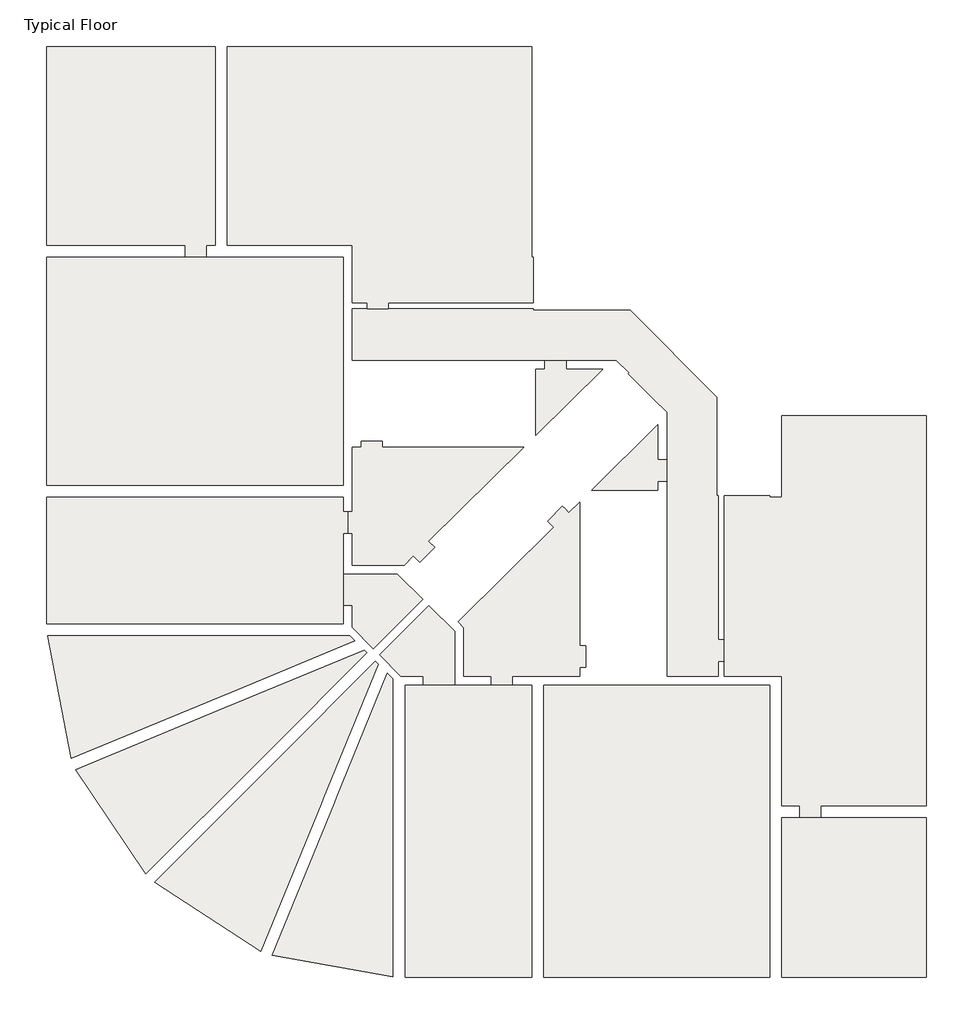
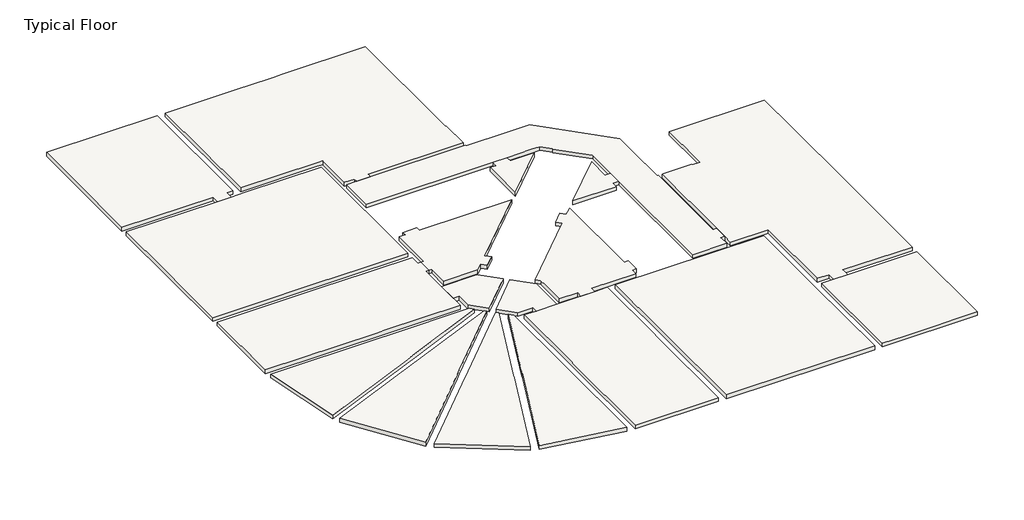
# One storey: 19 slabs.
"""IFC4 building model written with IfcOpenShell, lengths in millimetres."""

from ifc_helpers import new_model, si_unit, frame, origin, place, context, project, spatial, polyline, outline, extrude, faceted_brep, element, save

model = new_model("IFC4")

# Units and contexts
model_context = context("Model", 3, world=origin())
ifc_project = project(units=[si_unit("LENGTHUNIT", "METRE", prefix="MILLI")], contexts=[model_context])

# Site, building, storey
site = spatial("IfcSite", under=ifc_project)
building = spatial("IfcBuilding", under=site)
storey = spatial("IfcBuildingStorey", under=building, Name="Typical Floor", Elevation=3000.0)

# Slabs
placement = place(None, origin())
element("IfcSlab", 1, ObjectType="20", at=placement, inside=storey, context=model_context, shape_type="Brep", body=[
    faceted_brep([(-4461.7067397, 17456.8664083, 2800.0), (-4461.7067397, 9912.1590026, 2800.0), (-14296.6369988, 9912.1590026, 2800.0), (-14296.6369988, 17456.8664083, 2800.0), (-9693.3146493, 17456.8664083, 2800.0), (-9006.7279431, 17456.8664083, 2800.0), (-4461.7067397, 17456.8664083, 3000.0), (-8305.861308, 17456.8664083, 3000.0), (-9006.7279431, 17456.8664083, 3000.0), (-9693.3146493, 17456.8664083, 3000.0), (-14296.6369988, 17456.8664083, 3000.0), (-14296.6369988, 14107.3138675, 3000.0), (-14296.6369988, 13707.3138675, 3000.0), (-14296.6369988, 9912.1590026, 3000.0), (-8707.7294598, 9912.1590026, 3000.0), (-8307.7294598, 9912.1590026, 3000.0), (-4461.7067397, 9912.1590026, 3000.0)], [[[0, 1, 2, 3, 4, 5]], [[6, 7, 8, 9, 10, 11, 12, 13, 14, 15, 16]], [[1, 0, 6, 16]], [[2, 1, 16, 15, 14, 13]], [[3, 2, 13, 12, 11, 10]], [[0, 5, 4, 3, 10, 9, 8, 7, 6]]]),
])
element("IfcSlab", 2, ObjectType="20", at=placement, inside=storey, context=model_context, shape_type="SweptSolid", body=[
    extrude(outline(polyline([(-8705.861308, 24444.3058567), (-8705.861308, 17856.8664083), (-9006.7279431, 17856.8664083), (-9006.7279431, 17456.8664083), (-9693.3146493, 17456.8664083), (-9693.3146493, 17856.8664083), (-14296.6369988, 17856.8664083), (-14296.6369988, 24444.3058567), (-8705.861308, 24444.3058567)])), frame((0.0, 0.0, 2800.0), z_axis=(0.0, 0.0, 1.0), x_axis=(1.0, 0.0, 0.0)), (0.0, 0.0, 1.0), 200.0),
])
element("IfcSlab", 3, ObjectType="20", at=placement, inside=storey, context=model_context, shape_type="Brep", body=[
    faceted_brep([(1779.020722, 24445.393344, 2800.0), (1779.020722, 17856.8664083, 2800.0), (1779.020722, 17853.6134053, 2800.0), (1779.020722, 17453.6134053, 2800.0), (1829.020722, 17453.6134053, 2800.0), (1829.020722, 15961.3377606, 2800.0), (-2964.398431, 15961.3377606, 2800.0), (-2964.398431, 15761.3377606, 2800.0), (-3665.2660617, 15761.3377606, 2800.0), (-3665.2660617, 15961.3377606, 2800.0), (-4161.7067397, 15961.3377606, 2800.0), (-4161.7067397, 17856.8664083, 2800.0), (-4461.7067397, 17856.8664083, 2800.0), (-8305.861308, 17856.8664083, 2800.0), (-8305.861308, 24445.393344, 2800.0), (1779.020722, 17856.8664083, 3000.0), (1779.020722, 24445.393344, 3000.0), (-2413.8658054, 24445.393344, 3000.0), (-2813.8658054, 24445.393344, 3000.0), (-4118.3634455, 24445.393344, 3000.0), (-4518.3634455, 24445.393344, 3000.0), (-8305.861308, 24445.393344, 3000.0), (-8305.861308, 24444.3058567, 3000.0), (-8305.861308, 17856.8664083, 3000.0), (-4461.7067397, 17856.8664083, 3000.0), (-4161.7067397, 17856.8664083, 3000.0), (-4161.7067397, 15961.3377606, 3000.0), (-3665.2660617, 15961.3377606, 3000.0), (-3665.2660617, 15761.3377606, 3000.0), (-2964.398431, 15761.3377606, 3000.0), (-2964.398431, 15961.3377606, 3000.0), (1829.020722, 15961.3377606, 3000.0), (1829.020722, 16003.9996895, 3000.0), (1829.020722, 17453.6134053, 3000.0), (1779.020722, 17453.6134053, 3000.0), (1779.020722, 17853.6134053, 3000.0)], [[[0, 1, 2, 3, 4, 5, 6, 7, 8, 9, 10, 11, 12, 13, 14]], [[15, 16, 17, 18, 19, 20, 21, 22, 23, 24, 25, 26, 27, 28, 29, 30, 31, 32, 33, 34, 35]], [[1, 0, 16, 15]], [[1, 15, 35, 34, 3, 2]], [[4, 3, 34, 33]], [[5, 4, 33, 32, 31]], [[6, 5, 31, 30]], [[7, 6, 30, 29]], [[8, 7, 29, 28]], [[9, 8, 28, 27]], [[10, 9, 27, 26]], [[11, 10, 26, 25]], [[11, 25, 24, 23, 13, 12]], [[14, 13, 23, 22, 21]], [[0, 14, 21, 20, 19, 18, 17, 16]]]),
])
element("IfcSlab", 4, ObjectType="20", at=placement, inside=storey, context=model_context, shape_type="Brep", body=[
    faceted_brep([(-14296.6369988, 5319.511412, 2800.0), (-14296.6369988, 9512.1590026, 2800.0), (-4461.7067397, 9512.1590026, 2800.0), (-4461.7067397, 9032.3032318, 2800.0), (-4317.7621118, 9032.3032318, 2800.0), (-4317.7621118, 8319.3213117, 2800.0), (-4467.7621118, 8319.3213117, 2800.0), (-4467.7621118, 7259.3213117, 2800.0), (-4467.7621118, 6959.3213117, 2800.0), (-4467.7621118, 5921.5426188, 2800.0), (-4467.7621118, 5491.5426188, 2800.0), (-4467.7621118, 5319.511412, 2800.0), (-14296.6369988, 9512.1590026, 3000.0), (-14296.6369988, 5319.511412, 3000.0), (-8707.7294598, 5319.511412, 3000.0), (-8307.7294598, 5319.511412, 3000.0), (-4467.7621118, 5319.511412, 3000.0), (-4467.7621118, 5491.5426188, 3000.0), (-4467.7621118, 5921.5426188, 3000.0), (-4467.7621118, 6959.3213117, 3000.0), (-4467.7621118, 7259.3213117, 3000.0), (-4467.7621118, 8319.3213117, 3000.0), (-4317.7621118, 8319.3213117, 3000.0), (-4317.7621118, 9032.3032318, 3000.0), (-4461.7067397, 9032.3032318, 3000.0), (-4461.7067397, 9512.1590026, 3000.0), (-8307.7294598, 9512.1590026, 3000.0), (-8707.7294598, 9512.1590026, 3000.0)], [[[0, 1, 2, 3, 4, 5, 6, 7, 8, 9, 10, 11]], [[12, 13, 14, 15, 16, 17, 18, 19, 20, 21, 22, 23, 24, 25, 26, 27]], [[1, 0, 13, 12]], [[2, 1, 12, 27, 26, 25]], [[3, 2, 25, 24]], [[4, 3, 24, 23]], [[5, 4, 23, 22]], [[6, 5, 22, 21]], [[6, 21, 20, 19, 18, 9, 8, 7]], [[9, 18, 17, 16, 11, 10]], [[0, 11, 16, 15, 14, 13]]]),
])
element("IfcSlab", 5, ObjectType="20", at=placement, inside=storey, context=model_context, shape_type="Brep", body=[
    faceted_brep([(-4249.2842956, 4919.511412, 2800.0), (-4077.2097101, 4747.4368266, 2800.0), (-8177.5148344, 3048.7578016, 2800.0), (-8547.0578193, 2895.6631176, 2800.0), (-13484.0892311, 850.3441838, 2800.0), (-14261.3814687, 4919.511412, 2800.0), (-4077.2097101, 4747.4368266, 3000.0), (-4249.2842956, 4919.511412, 3000.0), (-8307.7294598, 4919.511412, 3000.0), (-8707.7294598, 4919.511412, 3000.0), (-14261.3814687, 4919.511412, 3000.0), (-13484.0892311, 850.3441838, 3000.0), (-8547.0578193, 2895.6631176, 3000.0), (-8177.5148344, 3048.7578016, 3000.0)], [[[0, 1, 2, 3, 4, 5]], [[6, 7, 8, 9, 10, 11, 12, 13]], [[1, 0, 7, 6]], [[1, 6, 13, 12, 11, 4, 3, 2]], [[5, 4, 11, 10]], [[0, 5, 10, 9, 8, 7]]]),
])
element("IfcSlab", 6, ObjectType="20", at=placement, inside=storey, context=model_context, shape_type="Brep", body=[
    faceted_brep([(-11001.7177394, -2970.8920309, 2800.0), (-13331.7826338, 480.4747094, 2800.0), (-8393.9631353, 2526.1201326, 2800.0), (-8024.4201504, 2679.2148167, 2800.0), (-3771.0702765, 4441.2973929, 2800.0), (-3680.299296, 4350.5264125, 2800.0), (-6954.3339133, 1076.4917952, 2800.0), (-7237.1766258, 793.6490827, 2800.0), (-13331.7826338, 480.4747094, 3000.0), (-11001.7177394, -2970.8920309, 3000.0), (-7237.1766258, 793.6490827, 3000.0), (-6954.3339133, 1076.4917952, 3000.0), (-3680.299296, 4350.5264125, 3000.0), (-3771.0702765, 4441.2973929, 3000.0), (-8024.4201504, 2679.2148167, 3000.0), (-8393.9631353, 2526.1201326, 3000.0)], [[[0, 1, 2, 3, 4, 5, 6, 7]], [[8, 9, 10, 11, 12, 13, 14, 15]], [[1, 0, 9, 8]], [[1, 8, 15, 14, 13, 4, 3, 2]], [[5, 4, 13, 12]], [[5, 12, 11, 10, 9, 0, 7, 6]]]),
])
element("IfcSlab", 7, ObjectType="20", at=placement, inside=storey, context=model_context, shape_type="Brep", body=[
    faceted_brep([(-3397.4447571, 4067.6718736, 2800.0), (-3302.3291451, 3972.5562616, 2800.0), (-5120.1129012, -471.1947368, 2800.0), (-5195.1092439, -649.6362255, 2800.0), (-5193.4008185, -650.3542517, 2800.0), (-7191.7801663, -5535.5889186, 2800.0), (-10715.1044827, -3249.987852, 2800.0), (-6954.3220945, 510.7945362, 2800.0), (-6671.4793821, 793.6372486, 2800.0), (-3302.3291451, 3972.5562616, 3000.0), (-3397.4447571, 4067.6718736, 3000.0), (-6671.4793821, 793.6372486, 3000.0), (-6954.3220945, 510.7945362, 3000.0), (-10715.1044827, -3249.987852, 3000.0), (-7191.7801663, -5535.5889186, 3000.0), (-5193.4008185, -650.3542517, 3000.0), (-5195.1092439, -649.6362255, 3000.0), (-5120.1129012, -471.1947368, 3000.0), (-5119.2358115, -469.0506048, 3000.0)], [[[0, 1, 2, 3, 4, 5, 6, 7, 8]], [[9, 10, 11, 12, 13, 14, 15, 16, 17, 18]], [[1, 0, 10, 9]], [[1, 9, 18, 17, 2]], [[14, 5, 4, 15]], [[6, 5, 14, 13]], [[6, 13, 12, 11, 10, 0, 8, 7]], [[3, 16, 15, 4]], [[16, 3, 2, 17]]]),
])
element("IfcSlab", 8, ObjectType="20", at=placement, inside=storey, context=model_context, shape_type="Brep", body=[
    faceted_brep([(-2813.8658054, 3484.0929218, 2800.0), (-2813.8658054, -6379.2217224, 2800.0), (-6818.4727302, -5679.49154, 2800.0), (-4750.6157411, -624.4119522, 2800.0), (-4671.3715454, -435.8633948, 2800.0), (-4673.1767374, -435.1046991, 2800.0), (-2995.6201329, 3665.8472494, 2800.0), (-2909.1120413, 3579.3391577, 2800.0), (-2813.8658054, -6379.2217224, 3000.0), (-2813.8658054, -1123.2844162, 3000.0), (-2813.8658054, -723.2844162, 3000.0), (-2813.8658054, 3484.0929218, 3000.0), (-2909.1120413, 3579.3391577, 3000.0), (-2995.6201329, 3665.8472494, 3000.0), (-4673.1767374, -435.1046991, 3000.0), (-4671.3715454, -435.8633948, 3000.0), (-4750.6157411, -624.4119522, 3000.0), (-6818.4727302, -5679.49154, 3000.0)], [[[0, 1, 2, 3, 4, 5, 6, 7]], [[8, 9, 10, 11, 12, 13, 14, 15, 16, 17]], [[1, 0, 11, 10, 9, 8]], [[2, 1, 8, 17]], [[13, 6, 5, 14]], [[2, 17, 16, 3]], [[6, 13, 12, 11, 0, 7]], [[4, 15, 14, 5]], [[15, 4, 3, 16]]]),
])
element("IfcSlab", 9, ObjectType="20", at=placement, inside=storey, context=model_context, shape_type="Brep", body=[
    faceted_brep([(1779.020722, 3279.3391577, 2800.0), (1779.020722, -6410.076772, 2800.0), (-2413.8658054, -6410.076772, 2800.0), (-2413.8658054, 3279.3391577, 2800.0), (-1817.5239543, 3279.3391577, 2800.0), (-769.9852407, 3279.3391577, 2800.0), (450.0147593, 3279.3391577, 2800.0), (1134.6168888, 3279.3391577, 2800.0), (1779.020722, 3279.3391577, 3000.0), (1134.6168888, 3279.3391577, 3000.0), (450.0147593, 3279.3391577, 3000.0), (-469.9852407, 3279.3391577, 3000.0), (-769.9852407, 3279.3391577, 3000.0), (-1817.5239543, 3279.3391577, 3000.0), (-2413.8658054, 3279.3391577, 3000.0), (-2413.8658054, -723.2844162, 3000.0), (-2413.8658054, -1123.2844162, 3000.0), (-2413.8658054, -6410.076772, 3000.0), (1779.020722, -6410.076772, 3000.0), (1779.020722, -1123.2844162, 3000.0), (1779.020722, -723.2844162, 3000.0)], [[[0, 1, 2, 3, 4, 5, 6, 7]], [[8, 9, 10, 11, 12, 13, 14, 15, 16, 17, 18, 19, 20]], [[1, 0, 8, 20, 19, 18]], [[2, 1, 18, 17]], [[3, 2, 17, 16, 15, 14]], [[0, 7, 6, 5, 4, 3, 14, 13, 12, 11, 10, 9, 8]]]),
])
element("IfcSlab", 10, ObjectType="20", at=placement, inside=storey, context=model_context, shape_type="Brep", body=[
    faceted_brep([(9669.6339123, 3279.3391577, 2800.0), (9669.6339123, -6410.076772, 2800.0), (2179.020722, -6410.076772, 2800.0), (2179.020722, 3279.3391577, 2800.0), (9669.6339123, 3279.3391577, 3000.0), (2179.020722, 3279.3391577, 3000.0), (2179.020722, -723.2844162, 3000.0), (2179.020722, -1123.2844162, 3000.0), (2179.020722, -6410.076772, 3000.0), (5922.4147884, -6410.076772, 3000.0), (6322.4147884, -6410.076772, 3000.0), (9669.6339123, -6410.076772, 3000.0), (9669.6339123, -1116.1309652, 3000.0), (9669.6339123, -716.1309652, 3000.0)], [[[0, 1, 2, 3]], [[4, 5, 6, 7, 8, 9, 10, 11, 12, 13]], [[1, 0, 4, 13, 12, 11]], [[2, 1, 11, 10, 9, 8]], [[3, 2, 8, 7, 6, 5]], [[0, 3, 5, 4]]]),
])
element("IfcSlab", 11, ObjectType="20", at=placement, inside=storey, context=model_context, shape_type="Brep", body=[
    faceted_brep([(14862.6652109, -1116.1309652, 2800.0), (14862.6652109, -6410.076772, 2800.0), (10069.6339123, -6410.076772, 2800.0), (10069.6339123, -1116.1309652, 2800.0), (10670.3228524, -1116.1309652, 2800.0), (11362.6652109, -1116.1309652, 2800.0), (14862.6652109, -1116.1309652, 3000.0), (11362.6652109, -1116.1309652, 3000.0), (10670.3228524, -1116.1309652, 3000.0), (10069.6339123, -1116.1309652, 3000.0), (10069.6339123, -6410.076772, 3000.0), (11162.4147884, -6410.076772, 3000.0), (14862.6652109, -6410.076772, 3000.0)], [[[0, 1, 2, 3, 4, 5]], [[6, 7, 8, 9, 10, 11, 12]], [[1, 0, 6, 12]], [[2, 1, 12, 11, 10]], [[3, 2, 10, 9]], [[0, 5, 4, 3, 9, 8, 7, 6]]]),
])
element("IfcSlab", 12, ObjectType="20", at=placement, inside=storey, context=model_context, shape_type="Brep", body=[
    faceted_brep([(10670.3228524, -716.1309652, 2800.0), (10069.6339123, -716.1309652, 2800.0), (10069.6339123, 3279.3391577, 2800.0), (10069.6339123, 3579.3391577, 2800.0), (8168.0773416, 3579.3391577, 2800.0), (8168.0773416, 4078.4432768, 2800.0), (8168.0773416, 4779.3109075, 2800.0), (8168.0773416, 9562.1590026, 2800.0), (8219.6339123, 9562.1590026, 2800.0), (9669.6339123, 9562.1590026, 2800.0), (9669.6339123, 9512.1590026, 2800.0), (10069.6339123, 9512.1590026, 2800.0), (10069.6339123, 9912.1590026, 2800.0), (10069.6339123, 12213.3492909, 2800.0), (14862.3806142, 12213.3492909, 2800.0), (14862.3806142, -716.1309652, 2800.0), (11362.6652109, -716.1309652, 2800.0), (11362.6652109, -1116.1309652, 2800.0), (10670.3228524, -1116.1309652, 2800.0), (10069.6339123, -716.1309652, 3000.0), (10670.3228524, -716.1309652, 3000.0), (10670.3228524, -1116.1309652, 3000.0), (11362.6652109, -1116.1309652, 3000.0), (11362.6652109, -716.1309652, 3000.0), (14862.3806142, -716.1309652, 3000.0), (14862.3806142, 3228.4489922, 3000.0), (14862.3806142, 3628.4489922, 3000.0), (14862.3806142, 4919.511412, 3000.0), (14862.3806142, 5319.511412, 3000.0), (14862.3806142, 9512.1590026, 3000.0), (14862.3806142, 9912.1590026, 3000.0), (14862.3806142, 12213.3492909, 3000.0), (10069.6339123, 12213.3492909, 3000.0), (10069.6339123, 9912.1590026, 3000.0), (10069.6339123, 9512.1590026, 3000.0), (9669.6339123, 9512.1590026, 3000.0), (9669.6339123, 9562.1590026, 3000.0), (8219.6339123, 9562.1590026, 3000.0), (8168.0773416, 9562.1590026, 3000.0), (8168.0773416, 4779.3109075, 3000.0), (8168.0773416, 4078.4432768, 3000.0), (8168.0773416, 3579.3391577, 3000.0), (10069.6339123, 3579.3391577, 3000.0), (10069.6339123, 3279.3391577, 3000.0)], [[[0, 1, 2, 3, 4, 5, 6, 7, 8, 9, 10, 11, 12, 13, 14, 15, 16, 17, 18]], [[19, 20, 21, 22, 23, 24, 25, 26, 27, 28, 29, 30, 31, 32, 33, 34, 35, 36, 37, 38, 39, 40, 41, 42, 43]], [[1, 0, 20, 19]], [[1, 19, 43, 42, 3, 2]], [[4, 3, 42, 41]], [[6, 5, 4, 41, 40, 39]], [[7, 6, 39, 38]], [[7, 38, 37, 36, 9, 8]], [[10, 9, 36, 35]], [[11, 10, 35, 34]], [[11, 34, 33, 32, 13, 12]], [[14, 13, 32, 31]], [[15, 14, 31, 30, 29, 28, 27, 26, 25, 24]], [[16, 15, 24, 23]], [[17, 16, 23, 22]], [[18, 17, 22, 21]], [[0, 18, 21, 20]]]),
])
element("IfcSlab", 13, ObjectType="20", at=placement, inside=storey, context=model_context, shape_type="SweptSolid", body=[
    extrude(outline(polyline([(-769.9852407, 5064.4841024), (-769.9852407, 3279.3391577), (-1817.5239543, 3279.3391577), (-1817.5239543, 3579.3391577), (-2555.5586507, 3579.3391577), (-3256.6787431, 4280.4592501), (-1621.3195657, 5915.8184274), (-769.9852407, 5064.4841024)])), frame((0.0, 0.0, 2800.0), z_axis=(0.0, 0.0, 1.0), x_axis=(1.0, 0.0, 0.0)), (0.0, 0.0, 1.0), 200.0),
])
element("IfcSlab", 14, ObjectType="20", at=placement, inside=storey, context=model_context, shape_type="Brep", body=[
    faceted_brep([(-2664.82245, 6959.3213117, 2800.0), (-1833.4516001, 6127.9504618, 2800.0), (-3468.8107774, 4492.5912844, 2800.0), (-4167.7621118, 5191.5426188, 2800.0), (-4167.7621118, 5921.5426188, 2800.0), (-4467.7621118, 5921.5426188, 2800.0), (-4467.7621118, 6959.3213117, 2800.0), (-1833.4516001, 6127.9504618, 3000.0), (-2664.82245, 6959.3213117, 3000.0), (-2752.523137, 6959.3213117, 3000.0), (-4467.7621118, 6959.3213117, 3000.0), (-4467.7621118, 5921.5426188, 3000.0), (-4167.7621118, 5921.5426188, 3000.0), (-4167.7621118, 5191.5426188, 3000.0), (-3468.8107774, 4492.5912844, 3000.0)], [[[0, 1, 2, 3, 4, 5, 6]], [[7, 8, 9, 10, 11, 12, 13, 14]], [[1, 0, 8, 7]], [[2, 1, 7, 14]], [[3, 2, 14, 13]], [[4, 3, 13, 12]], [[5, 4, 12, 11]], [[6, 5, 11, 10]], [[0, 6, 10, 9, 8]]]),
])
element("IfcSlab", 15, ObjectType="20", at=placement, inside=storey, context=model_context, shape_type="SweptSolid", body=[
    extrude(outline(polyline([(-4317.7621118, 9032.3032318), (-4161.7067397, 9032.3032318), (-4161.7067397, 11166.7645142), (-3861.7208648, 11166.7645142), (-3861.7208648, 11366.7645142), (-3166.1629714, 11366.7645142), (-3166.1629714, 11166.7645142), (1521.6521635, 11166.7645142), (-1638.9943721, 8055.4647086), (-1428.5378745, 7841.6702684), (-1923.597057, 7354.3403753), (-2134.0535546, 7568.1348155), (-2447.7649909, 7259.3213117), (-4167.7621118, 7259.3213117), (-4167.7621118, 8319.3213117), (-4317.7621118, 8319.3213117), (-4317.7621118, 9032.3032318)])), frame((0.0, 0.0, 2800.0), z_axis=(0.0, 0.0, 1.0), x_axis=(1.0, 0.0, 0.0)), (0.0, 0.0, 1.0), 200.0),
])
element("IfcSlab", 16, ObjectType="20", at=placement, inside=storey, context=model_context, shape_type="Brep", body=[
    faceted_brep([(450.0147593, 3579.3391577, 2800.0), (-469.9852407, 3579.3391577, 2800.0), (-469.9852407, 4764.4841024, 2800.0), (-469.9852407, 5188.7481711, 2800.0), (-654.972774, 5373.7357044, 2800.0), (2521.8013373, 8504.6910362, 2800.0), (2309.6637065, 8716.8286669, 2800.0), (2804.6384533, 9211.8034138, 2800.0), (2897.8940684, 9118.5477987, 2800.0), (3019.4754557, 8995.1871747, 2800.0), (3020.3715361, 8996.0703309, 2800.0), (3375.2686355, 9345.8487309, 2800.0), (3375.2686355, 4577.5453716, 2800.0), (3575.2686355, 4577.5453716, 2800.0), (3575.2686355, 3876.6777409, 2800.0), (3375.2686355, 3876.6777409, 2800.0), (3375.2686355, 3579.3391577, 2800.0), (1134.6168888, 3579.3391577, 2800.0), (1134.6168888, 3279.3391577, 2800.0), (450.0147593, 3279.3391577, 2800.0), (-469.9852407, 3579.3391577, 3000.0), (450.0147593, 3579.3391577, 3000.0), (450.0147593, 3279.3391577, 3000.0), (1134.6168888, 3279.3391577, 3000.0), (1134.6168888, 3579.3391577, 3000.0), (3375.2686355, 3579.3391577, 3000.0), (3375.2686355, 3876.6777409, 3000.0), (3575.2686355, 3876.6777409, 3000.0), (3575.2686355, 4577.5453716, 3000.0), (3375.2686355, 4577.5453716, 3000.0), (3375.2686355, 9345.8487309, 3000.0), (3020.3715361, 8996.0703309, 3000.0), (3019.4754557, 8995.1871747, 3000.0), (2897.8940684, 9118.5477987, 3000.0), (2804.6384533, 9211.8034138, 3000.0), (2309.6637065, 8716.8286669, 3000.0), (2521.8013373, 8504.6910362, 3000.0), (-654.972774, 5373.7357044, 3000.0), (-469.9852407, 5188.7481711, 3000.0), (-469.9852407, 4764.4841024, 3000.0)], [[[0, 1, 2, 3, 4, 5, 6, 7, 8, 9, 10, 11, 12, 13, 14, 15, 16, 17, 18, 19]], [[20, 21, 22, 23, 24, 25, 26, 27, 28, 29, 30, 31, 32, 33, 34, 35, 36, 37, 38, 39]], [[1, 0, 21, 20]], [[1, 20, 39, 38, 3, 2]], [[4, 3, 38, 37]], [[5, 4, 37, 36]], [[6, 5, 36, 35]], [[7, 6, 35, 34]], [[7, 34, 33, 8]], [[29, 12, 11, 30]], [[13, 12, 29, 28]], [[14, 13, 28, 27]], [[15, 14, 27, 26]], [[16, 15, 26, 25]], [[17, 16, 25, 24]], [[18, 17, 24, 23]], [[19, 18, 23, 22]], [[0, 19, 22, 21]], [[9, 32, 31, 30, 11, 10]], [[32, 9, 8, 33]]]),
])
element("IfcSlab", 17, ObjectType="20", at=placement, inside=storey, context=model_context, shape_type="SweptSolid", body=[
    extrude(outline(polyline([(1924.8242608, 13749.3760398), (2223.0854171, 13749.3760398), (2223.0854171, 14049.3760398), (2926.3637213, 14049.3760398), (2926.3637213, 13749.3760398), (4145.2251653, 13749.3760398), (1924.8242608, 11563.6419424), (1924.8242608, 13749.3760398)])), frame((0.0, 0.0, 2800.0), z_axis=(0.0, 0.0, 1.0), x_axis=(1.0, 0.0, 0.0)), (0.0, 0.0, 1.0), 200.0),
])
element("IfcSlab", 18, ObjectType="20", at=placement, inside=storey, context=model_context, shape_type="SweptSolid", body=[
    extrude(outline(polyline([(5969.003497, 11902.1740186), (5969.003497, 10741.9965509), (6269.003497, 10741.9965509), (6269.003497, 10041.1289202), (5969.003497, 10041.1289202), (5969.003497, 9742.8632028), (3778.0930653, 9742.8632028), (5969.003497, 11902.1740186)])), frame((0.0, 0.0, 2800.0), z_axis=(0.0, 0.0, 1.0), x_axis=(1.0, 0.0, 0.0)), (0.0, 0.0, 1.0), 200.0),
])
element("IfcSlab", 19, ObjectType="20", at=placement, inside=storey, context=model_context, shape_type="Brep", body=[
    faceted_brep([(7968.0773416, 3579.3391577, 2800.0), (6269.003497, 3579.3391577, 2800.0), (6269.003497, 10041.1289202, 2800.0), (6269.003497, 10741.9965509, 2800.0), (6269.003497, 11899.9963547, 2800.0), (6269.003497, 12324.2604234, 2800.0), (5836.2714262, 12756.9924943, 2800.0), (4989.3898697, 13603.8740507, 2800.0), (5010.62779, 13625.111971, 2800.0), (4586.3637213, 14049.3760398, 2800.0), (4162.0996526, 14049.3760398, 2800.0), (2926.3637213, 14049.3760398, 2800.0), (2223.0854171, 14049.3760398, 2800.0), (-4161.7067397, 14049.3760398, 2800.0), (-4161.7067397, 15761.3377606, 2800.0), (-3665.2660617, 15761.3377606, 2800.0), (-2964.398431, 15761.3377606, 2800.0), (1829.020722, 15761.3377606, 2800.0), (1829.020722, 15703.9996895, 2800.0), (2129.020722, 15703.9996895, 2800.0), (3673.883474, 15703.9996895, 2800.0), (3973.883474, 15703.9996895, 2800.0), (5042.5813574, 15703.9996895, 2800.0), (7919.6339123, 12826.9471346, 2800.0), (7919.6339123, 11715.5910733, 2800.0), (7919.6339123, 11415.5910733, 2800.0), (7919.6339123, 9862.1590026, 2800.0), (7919.6339123, 9562.1590026, 2800.0), (7968.0773416, 9562.1590026, 2800.0), (7968.0773416, 4779.3109075, 2800.0), (8168.0773416, 4779.3109075, 2800.0), (8168.0773416, 4078.4432768, 2800.0), (7968.0773416, 4078.4432768, 2800.0), (6269.003497, 3579.3391577, 3000.0), (7968.0773416, 3579.3391577, 3000.0), (7968.0773416, 4078.4432768, 3000.0), (8168.0773416, 4078.4432768, 3000.0), (8168.0773416, 4779.3109075, 3000.0), (7968.0773416, 4779.3109075, 3000.0), (7968.0773416, 9562.1590026, 3000.0), (7919.6339123, 9562.1590026, 3000.0), (7919.6339123, 9862.1590026, 3000.0), (7919.6339123, 11415.5910733, 3000.0), (7919.6339123, 11715.5910733, 3000.0), (7919.6339123, 12826.9471346, 3000.0), (5042.5813574, 15703.9996895, 3000.0), (3973.883474, 15703.9996895, 3000.0), (3673.883474, 15703.9996895, 3000.0), (2129.020722, 15703.9996895, 3000.0), (1829.020722, 15703.9996895, 3000.0), (1829.020722, 15761.3377606, 3000.0), (-2964.398431, 15761.3377606, 3000.0), (-3665.2660617, 15761.3377606, 3000.0), (-4161.7067397, 15761.3377606, 3000.0), (-4161.7067397, 14049.3760398, 3000.0), (2223.0854171, 14049.3760398, 3000.0), (2926.3637213, 14049.3760398, 3000.0), (4162.0996526, 14049.3760398, 3000.0), (4586.3637213, 14049.3760398, 3000.0), (5010.62779, 13625.111971, 3000.0), (4989.3898697, 13603.8740507, 3000.0), (5836.2714262, 12756.9924943, 3000.0), (6269.003497, 12324.2604234, 3000.0), (6269.003497, 11899.9963547, 3000.0), (6269.003497, 10741.9965509, 3000.0), (6269.003497, 10041.1289202, 3000.0)], [[[0, 1, 2, 3, 4, 5, 6, 7, 8, 9, 10, 11, 12, 13, 14, 15, 16, 17, 18, 19, 20, 21, 22, 23, 24, 25, 26, 27, 28, 29, 30, 31, 32]], [[33, 34, 35, 36, 37, 38, 39, 40, 41, 42, 43, 44, 45, 46, 47, 48, 49, 50, 51, 52, 53, 54, 55, 56, 57, 58, 59, 60, 61, 62, 63, 64, 65]], [[1, 0, 34, 33]], [[1, 33, 65, 64, 63, 62, 5, 4, 3, 2]], [[5, 62, 61, 60, 7, 6]], [[8, 7, 60, 59]], [[9, 8, 59, 58]], [[9, 58, 57, 56, 55, 54, 13, 12, 11, 10]], [[14, 13, 54, 53]], [[17, 16, 15, 14, 53, 52, 51, 50]], [[18, 17, 50, 49]], [[18, 49, 48, 47, 46, 45, 22, 21, 20, 19]], [[40, 27, 26, 25, 24, 23, 44, 43, 42, 41]], [[28, 27, 40, 39]], [[29, 28, 39, 38]], [[23, 22, 45, 44]], [[30, 29, 38, 37]], [[31, 30, 37, 36]], [[32, 31, 36, 35]], [[0, 32, 35, 34]]]),
])

save(model, "model.ifc")

# Revit data of these elements
# Type "20"
#   Function = 0
#   Layers, outside or top first: 20 cm "Concrete" (function 1)
# Element 1 (IfcSlab, "20")
#   Mark = "S1"
#   SOFiSTiK_AMG_Comments = ""
#   Height Offset From Level = 0 cm
#   built-in parameter 1001954 = 1
#   SOFiSTiK_AMG_Scheduled = yes
#   SOFiSTiK_AMG_Adjusted = yes
#   Phase Created = New Construction
#   Materials on its faces: "Concrete"
# Element 2 (IfcSlab, "20")
#   Mark = "S2"
#   SOFiSTiK_AMG_Comments = ""
#   Height Offset From Level = 0 cm
#   built-in parameter 1001954 = 1
#   SOFiSTiK_AMG_Scheduled = yes
#   SOFiSTiK_AMG_Adjusted = yes
#   Phase Created = New Construction
#   Materials on its faces: "Concrete"
# Element 3 (IfcSlab, "20")
#   Mark = "S3"
#   SOFiSTiK_AMG_Comments = ""
#   Height Offset From Level = 0 cm
#   built-in parameter 1001954 = 1
#   SOFiSTiK_AMG_Scheduled = yes
#   SOFiSTiK_AMG_Adjusted = yes
#   Phase Created = New Construction
#   Materials on its faces: "Concrete"
# Element 4 (IfcSlab, "20")
#   Mark = "S4"
#   SOFiSTiK_AMG_Comments = ""
#   built-in parameter 1001955 = -1.5708 (stored number, unit not read)
#   Height Offset From Level = 0 cm
#   built-in parameter 1001954 = 1
#   SOFiSTiK_AMG_Scheduled = yes
#   SOFiSTiK_AMG_Adjusted = yes
#   Phase Created = New Construction
#   Materials on its faces: "Concrete"
# Element 5 (IfcSlab, "20")
#   Mark = "S5"
#   SOFiSTiK_AMG_Comments = ""
#   Height Offset From Level = 0 cm
#   built-in parameter 1001954 = 1
#   SOFiSTiK_AMG_Scheduled = yes
#   SOFiSTiK_AMG_Adjusted = yes
#   Phase Created = New Construction
#   Materials on its faces: "Concrete"
# Element 6 (IfcSlab, "20")
#   Mark = "S6"
#   SOFiSTiK_AMG_Comments = ""
#   built-in parameter 1001955 = -0.976969 (stored number, unit not read)
#   Height Offset From Level = 0 cm
#   built-in parameter 1001954 = 1
#   SOFiSTiK_AMG_Scheduled = yes
#   SOFiSTiK_AMG_Adjusted = yes
#   Phase Created = New Construction
#   Materials on its faces: "Concrete"
# Element 7 (IfcSlab, "20")
#   Mark = "S7"
#   SOFiSTiK_AMG_Comments = ""
#   built-in parameter 1001955 = 2.35619 (stored number, unit not read)
#   Height Offset From Level = 0 cm
#   built-in parameter 1001954 = 1
#   SOFiSTiK_AMG_Scheduled = yes
#   SOFiSTiK_AMG_Adjusted = yes
#   Phase Created = New Construction
#   Materials on its faces: "Concrete"
# Element 8 (IfcSlab, "20")
#   Mark = "S8"
#   SOFiSTiK_AMG_Comments = ""
#   built-in parameter 1001955 = -0.785398 (stored number, unit not read)
#   Height Offset From Level = 0 cm
#   built-in parameter 1001954 = 1
#   SOFiSTiK_AMG_Scheduled = yes
#   SOFiSTiK_AMG_Adjusted = yes
#   Phase Created = New Construction
#   Materials on its faces: "Concrete"
# Element 9 (IfcSlab, "20")
#   Mark = "S9"
#   SOFiSTiK_AMG_Comments = ""
#   Height Offset From Level = 0 cm
#   built-in parameter 1001954 = 1
#   SOFiSTiK_AMG_Scheduled = yes
#   SOFiSTiK_AMG_Adjusted = yes
#   Phase Created = New Construction
#   Materials on its faces: "Concrete"
# Element 10 (IfcSlab, "20")
#   Mark = "S10"
#   SOFiSTiK_AMG_Comments = ""
#   Height Offset From Level = 0 cm
#   built-in parameter 1001954 = 1
#   SOFiSTiK_AMG_Scheduled = yes
#   SOFiSTiK_AMG_Adjusted = yes
#   Phase Created = New Construction
#   Materials on its faces: "Concrete"
# Element 11 (IfcSlab, "20")
#   Mark = "S11"
#   SOFiSTiK_AMG_Comments = ""
#   Height Offset From Level = 0 cm
#   built-in parameter 1001954 = 1
#   SOFiSTiK_AMG_Scheduled = yes
#   SOFiSTiK_AMG_Adjusted = yes
#   Phase Created = New Construction
#   Materials on its faces: "Concrete"
# Element 12 (IfcSlab, "20")
#   Mark = "S12"
#   SOFiSTiK_AMG_Comments = ""
#   built-in parameter 1001955 = 1.5708 (stored number, unit not read)
#   Height Offset From Level = 0 cm
#   built-in parameter 1001954 = 1
#   SOFiSTiK_AMG_Scheduled = yes
#   SOFiSTiK_AMG_Adjusted = no
#   Phase Created = New Construction
#   Materials on its faces: "Concrete"
# Element 13 (IfcSlab, "20")
#   Mark = "S13"
#   SOFiSTiK_AMG_Comments = ""
#   built-in parameter 1001955 = 1.5708 (stored number, unit not read)
#   Height Offset From Level = 0 cm
#   built-in parameter 1001954 = 1
#   SOFiSTiK_AMG_Scheduled = yes
#   SOFiSTiK_AMG_Adjusted = yes
#   Phase Created = New Construction
#   Materials on its faces: "Concrete"
# Element 14 (IfcSlab, "20")
#   Mark = "S14"
#   SOFiSTiK_AMG_Comments = ""
#   Height Offset From Level = 0 cm
#   built-in parameter 1001954 = 1
#   SOFiSTiK_AMG_Scheduled = yes
#   SOFiSTiK_AMG_Adjusted = yes
#   Phase Created = New Construction
#   Materials on its faces: "Concrete"
# Element 15 (IfcSlab, "20")
#   Mark = "S15"
#   SOFiSTiK_AMG_Comments = ""
#   built-in parameter 1001955 = 1.5708 (stored number, unit not read)
#   Height Offset From Level = 0 cm
#   built-in parameter 1001954 = 1
#   SOFiSTiK_AMG_Scheduled = yes
#   SOFiSTiK_AMG_Adjusted = yes
#   Phase Created = New Construction
#   Materials on its faces: "Concrete"
# Element 16 (IfcSlab, "20")
#   Mark = "S16"
#   SOFiSTiK_AMG_Comments = ""
#   built-in parameter 1001955 = 1.5708 (stored number, unit not read)
#   Height Offset From Level = 0 cm
#   built-in parameter 1001954 = 1
#   SOFiSTiK_AMG_Scheduled = yes
#   SOFiSTiK_AMG_Adjusted = yes
#   Phase Created = New Construction
#   Materials on its faces: "Concrete"
# Element 17 (IfcSlab, "20")
#   Mark = "S17"
#   SOFiSTiK_AMG_Comments = ""
#   built-in parameter 1001955 = 0.77753 (stored number, unit not read)
#   Height Offset From Level = 0 cm
#   built-in parameter 1001954 = 1
#   SOFiSTiK_AMG_Scheduled = yes
#   SOFiSTiK_AMG_Adjusted = yes
#   Phase Created = New Construction
#   Materials on its faces: "Concrete"
# Element 18 (IfcSlab, "20")
#   Mark = "S18"
#   SOFiSTiK_AMG_Comments = ""
#   built-in parameter 1001955 = 0.778134 (stored number, unit not read)
#   Height Offset From Level = 0 cm
#   built-in parameter 1001954 = 1
#   SOFiSTiK_AMG_Scheduled = yes
#   SOFiSTiK_AMG_Adjusted = yes
#   Phase Created = New Construction
#   Materials on its faces: "Concrete"
# Element 19 (IfcSlab, "20")
#   Mark = "S19"
#   SOFiSTiK_AMG_Comments = ""
#   built-in parameter 1001955 = 0 (stored number, unit not read)
#   Height Offset From Level = 0 cm
#   built-in parameter 1001954 = 1
#   SOFiSTiK_AMG_Scheduled = yes
#   SOFiSTiK_AMG_Adjusted = yes
#   Phase Created = New Construction
#   Materials on its faces: "Concrete"
# Materials
#   "Concrete": class "Concrete", colour RGB 192 192 192, transparency 0, Keynote = "01000", Description = "Cast-in-place concrete", Cost = 0
